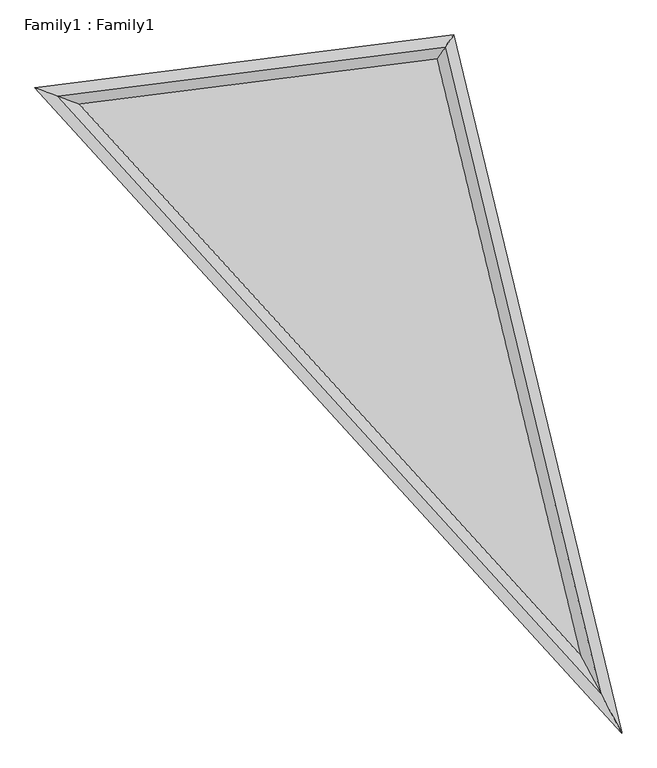
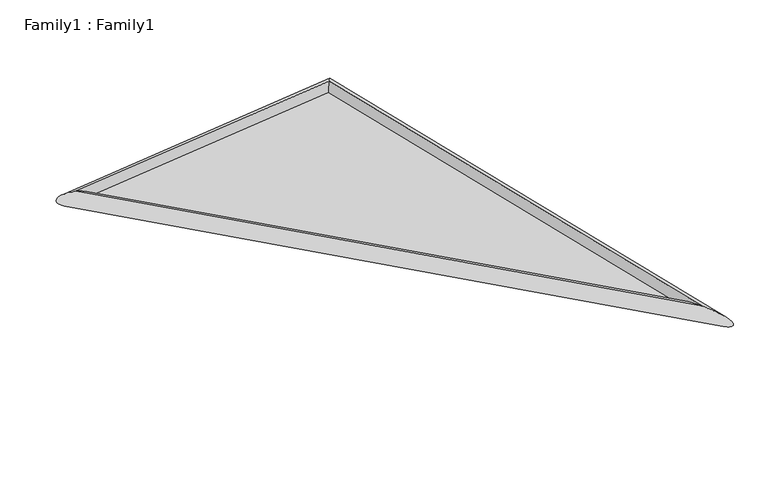
"""IFC4 building model written with IfcOpenShell, lengths in millimetres: proxy geometry, Family1 : Family1."""

from ifc_helpers import new_model, si_unit, frame, origin, origin_with_axes, place, context, project, spatial, polyline, ellipse_curve, outline, extrude, source, transform, mapped, element, save
from ifc_brep_helpers import cylinder_surface, advanced_brep


def family1_family1_2c3b855d(model_context):
    return source(origin(), model_context, "Body", "SolidModel", [
        extrude(outline(polyline([(3005.8714316, -3245.6856734), (-1852.77637, 2096.0904051), (1613.8273894, 2533.5364732), (3005.8714316, -3245.6856734)])), origin_with_axes(), (0.0, 0.0, 1.0), 34.1328789),
        advanced_brep(
        [(3005.8714316, -3245.6856734, 100.0), (3005.8714316, -3245.6856734, -100.0), (-1852.77637, 2096.0904051, -100.0), (-1852.77637, 2096.0904051, 100.0), (1613.8273894, 2533.5364732, -100.0), (1613.8273894, 2533.5364732, 100.0)],
        [
            (0, 1, ellipse_curve(frame((3005.8714316, -3245.6856734, 0.0), z_axis=(-0.8836382841936006, -0.4681702497034489, 0.0), x_axis=(0.46817024970344884, -0.8836382841936005, 0.0)), 402.8546968, 100.0)),
            (1, 2),
            (2, 3, ellipse_curve(frame((-1852.77637, 2096.0904051, 0.0), z_axis=(-0.34627786013033734, -0.9381319968871942, 0.0), x_axis=(0.9381319968871943, -0.3462778601303374, 0.0)), 216.918065, 100.0)),
            (3, 0),
            (1, 0, ellipse_curve(frame((3005.8714316, -3245.6856734, 0.0), z_axis=(-0.8836382841936006, -0.4681702497034489, 0.0), x_axis=(0.46817024970344884, -0.8836382841936005, 0.0)), 402.8546968, 100.0)),
            (3, 2, ellipse_curve(frame((-1852.77637, 2096.0904051, 0.0), z_axis=(-0.34627786013033734, -0.9381319968871942, 0.0), x_axis=(0.9381319968871943, -0.3462778601303374, 0.0)), 216.918065, 100.0)),
            (2, 4),
            (4, 5, ellipse_curve(frame((1613.8273894, 2533.5364732, 0.0), z_axis=(-0.8228138712979115, 0.5683109476331982, 0.0), x_axis=(-0.5683109476331984, -0.8228138712979114, 0.0)), 134.1939882, 100.0)),
            (5, 3),
            (5, 4, ellipse_curve(frame((1613.8273894, 2533.5364732, 0.0), z_axis=(-0.8228138712979115, 0.5683109476331982, 0.0), x_axis=(-0.5683109476331984, -0.8228138712979114, 0.0)), 134.1939882, 100.0)),
            (4, 1),
            (0, 5),
        ],
        [
            cylinder_surface(frame((3005.8714316, -3245.6856734, 0.0), z_axis=(0.6728614003187228, -0.7397685691898025, 0.0), x_axis=(-0.7397685691898025, -0.6728614003187228, 0.0)), 100.0),
            cylinder_surface(frame((-1852.77637, 2096.0904051, 0.0), z_axis=(-0.9921320522905688, -0.1251958099047412, 0.0), x_axis=(-0.1251958099047412, 0.9921320522905688, 0.0)), 100.0),
            cylinder_surface(frame((1613.8273894, 2533.5364732, 0.0), z_axis=(-0.2341730637413478, 0.9721949270686361, 0.0), x_axis=(0.9721949270686361, 0.2341730637413478, 0.0)), 100.0),
        ],
        [
            (0, [[1, 2, 3, 4]]),
            (0, [[5, -4, 6, -2]]),
            (1, [[-3, 7, 8, 9]]),
            (1, [[-6, -9, 10, -7]]),
            (2, [[-8, 11, -1, 12]]),
            (2, [[-10, -12, -5, -11]]),
        ],
    ),
    ])


if __name__ == "__main__":
    model = new_model("IFC4")
    model_context = context("Model", 3, world=origin())
    ifc_project = project(units=[si_unit("LENGTHUNIT", "METRE", prefix="MILLI")], contexts=[model_context])
    site = spatial("IfcSite", under=ifc_project)
    building = spatial("IfcBuilding", under=site)
    placement = place(None, origin())
    family1_family1_shape = family1_family1_2c3b855d(model_context)
    element("IfcBuildingElementProxy", 1, Name="Family1 : Family1", ObjectType="Family1 : Family1", at=placement, inside=building, context=model_context, shape_type="MappedRepresentation", body=[
        mapped(family1_family1_shape, transform((0.0, 0.0, 0.0), x_axis=(1.0, 0.0, 0.0), y_axis=(0.0, 1.0, 0.0), z_axis=(0.0, 0.0, 1.0))),
    ])
    save(model, "model.ifc")

# Revit data of these elements
# Type "Family1 : Family1"
#   Default Elevation = 0
# Element 1 (IfcBuildingElementProxy, "Family1 : Family1")
#   Materials on its faces: "Glass"
# Materials
#   "Glass": class "Glass", colour RGB 0 128 192, transparency 0.9, Description = "Soda Lime Glass", Cost = 0
